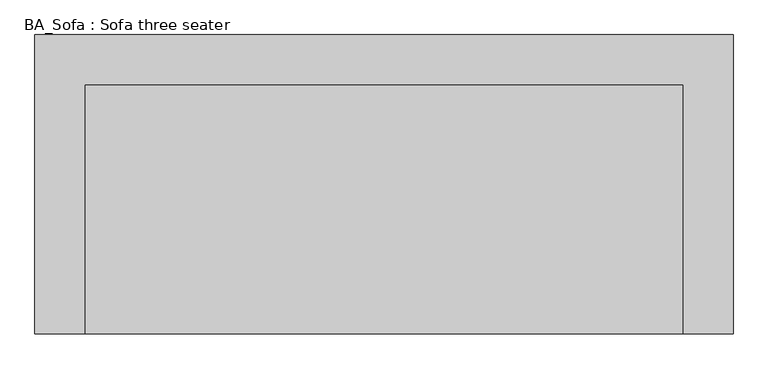
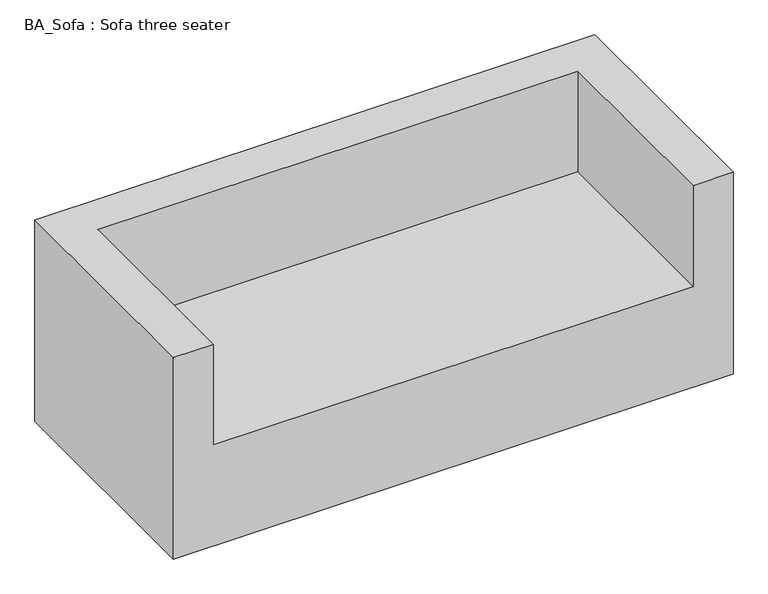
"""IFC4 building model written with IfcOpenShell, lengths in millimetres: furniture geometry, BA_Sofa : Sofa three seater."""

import ifcopenshell
import ifcopenshell.guid

model = None  # the IFC model being written
_history = None  # IfcOwnerHistory: only IFC2X3 demands one
_inside = {}  # id of a spatial element -> (the spatial element, [elements in it])
_under = {}  # id of a project, library or spatial element -> (it, [spatial elements below it])
_declared = {}  # id of a project -> (the project, [libraries it declares])
_typed = {}  # id of a type object -> (the type object, [elements of that type])
_made_of = {}  # id of a material, layer set ... -> (it, [elements and type objects made of it])


def new_model(schema):
    """Start an empty IFC model of exactly this schema.

    Asked for "IFC4X3", IfcOpenShell would pick the latest addendum, in which some entities
    have other attributes; the version numbers below select the first issue.
    IFC2X3 requires an IfcOwnerHistory on every rooted entity: one is made here for all.
    """
    global model, _history
    if schema == "IFC4X3":
        model = ifcopenshell.file(schema_version=(4, 3, 0, 0))
    else:
        model = ifcopenshell.file(schema=schema)
    _inside.clear()
    _under.clear()
    _declared.clear()
    _typed.clear()
    _made_of.clear()
    _history = None
    if model.schema == "IFC2X3":
        org = make("IfcOrganization", Name="unknown")
        user = make(
            "IfcPersonAndOrganization",
            ThePerson=make("IfcPerson", FamilyName="unknown"),
            TheOrganization=org,
        )
        app = make(
            "IfcApplication",
            ApplicationDeveloper=org,
            Version="unknown",
            ApplicationFullName="unknown",
            ApplicationIdentifier="unknown",
        )
        _history = make(
            "IfcOwnerHistory",
            OwningUser=user,
            OwningApplication=app,
            ChangeAction="ADDED",
            CreationDate=0,
        )
    return model


def make(cls, **values):
    """One entity of the class cls with the attributes given. An attribute that is None is left unset."""
    return model.create_entity(
        cls, **{name: value for name, value in values.items() if value is not None}
    )


def rooted(cls, **values):
    """An entity with a GlobalId (a new one), such as an element, a storey or a relation."""
    return make(cls, GlobalId=ifcopenshell.guid.new(), OwnerHistory=_history, **values)


def si_unit(unit_type, name, prefix=None):
    """IfcSIUnit, for example si_unit("LENGTHUNIT", "METRE", prefix="MILLI")."""
    return make("IfcSIUnit", UnitType=unit_type, Prefix=prefix, Name=name)


def assignment(units):
    """IfcUnitAssignment: the units of a project."""
    return None if units is None else make("IfcUnitAssignment", Units=units)


def point(xyz):
    """IfcCartesianPoint."""
    return None if xyz is None else make("IfcCartesianPoint", Coordinates=xyz)


def direction(xyz):
    """IfcDirection."""
    return None if xyz is None else make("IfcDirection", DirectionRatios=xyz)


def frame(location, z_axis=None, x_axis=None):
    """IfcAxis2Placement3D, a coordinate frame: its origin and axes. An axis left out is left unset."""
    return make(
        "IfcAxis2Placement3D",
        Location=point(location),
        Axis=direction(z_axis),
        RefDirection=direction(x_axis),
    )


def origin():
    """The frame at (0, 0, 0) with its axes left unset."""
    return frame((0.0, 0.0, 0.0))


def place(relative_to, where):
    """IfcLocalPlacement: puts the frame where relative to a parent placement (None: the world)."""
    return make(
        "IfcLocalPlacement", PlacementRelTo=relative_to, RelativePlacement=where
    )


def context(
    kind, dimensions, precision=None, world=None, true_north=None, identifier=None
):
    """IfcGeometricRepresentationContext, for example the 3D "Model" context."""
    return make(
        "IfcGeometricRepresentationContext",
        ContextIdentifier=identifier,
        ContextType=kind,
        CoordinateSpaceDimension=dimensions,
        Precision=precision,
        WorldCoordinateSystem=world,
        TrueNorth=true_north,
    )


def project(units=None, contexts=None):
    """IfcProject with its units and contexts."""
    return rooted(
        "IfcProject",
        Name="project",
        RepresentationContexts=contexts,
        UnitsInContext=assignment(units),
    )


def spatial(cls, under=None, at=None, **own):
    """A site, building, storey or space (cls), placed at a placement, below another one or the project."""
    s = rooted(cls, ObjectPlacement=at, **own)
    if under is not None:
        _under.setdefault(under.id(), (under, []))[1].append(s)
    return s


def faces_of(points, faces, orient=None, outer=None):
    """IfcFace entities. A face is a list of loops; a loop is a list of indices into points, from 0.

    orient and outer hold one flag for each loop. By default every Orientation is true, the
    first loop of a face is its IfcFaceOuterBound and the others are IfcFaceBound.
    """
    made = []
    for i, loops in enumerate(faces):
        bounds = []
        for j, loop in enumerate(loops):
            is_outer = j == 0 if outer is None else outer[i][j]
            bounds.append(
                make(
                    "IfcFaceOuterBound" if is_outer else "IfcFaceBound",
                    Bound=make("IfcPolyLoop", Polygon=[points[k] for k in loop]),
                    Orientation=True if orient is None else orient[i][j],
                )
            )
        made.append(make("IfcFace", Bounds=bounds))
    return made


def faceted_brep(points, faces, orient=None, outer=None, voids=None):
    """IfcFacetedBrep: a solid bounded by flat faces; with voids (closed shells), ...WithVoids."""
    shared = [point(p) for p in points]
    hull = make("IfcClosedShell", CfsFaces=faces_of(shared, faces, orient, outer))
    if voids is None:
        return make("IfcFacetedBrep", Outer=hull)
    return make(
        "IfcFacetedBrepWithVoids",
        Outer=hull,
        Voids=[
            make(cls, CfsFaces=faces_of(shared, fs, o, b)) for cls, fs, o, b in voids
        ],
    )


def shape(context_of_items, identifier, shape_type, items):
    """IfcShapeRepresentation: the items that make up one representation, for example the "Body"."""
    return make(
        "IfcShapeRepresentation",
        ContextOfItems=context_of_items,
        RepresentationIdentifier=identifier,
        RepresentationType=shape_type,
        Items=items,
    )


def source(mapping_origin, context_of_items, identifier, shape_type, items):
    """IfcRepresentationMap: a shape defined once, which mapped items show again and again."""
    return make(
        "IfcRepresentationMap",
        MappingOrigin=mapping_origin,
        MappedRepresentation=shape(context_of_items, identifier, shape_type, items),
    )


def transform(
    local_origin,
    x_axis=None,
    y_axis=None,
    z_axis=None,
    scale=None,
    scale2=None,
    scale3=None,
    uniform=True,
):
    """IfcCartesianTransformationOperator3D, or its non-uniform kind. x_axis, y_axis, z_axis: its Axis1, 2, 3."""
    if uniform:
        return make(
            "IfcCartesianTransformationOperator3D",
            Axis1=direction(x_axis),
            Axis2=direction(y_axis),
            LocalOrigin=point(local_origin),
            Scale=scale,
            Axis3=direction(z_axis),
        )
    return make(
        "IfcCartesianTransformationOperator3DnonUniform",
        Axis1=direction(x_axis),
        Axis2=direction(y_axis),
        LocalOrigin=point(local_origin),
        Scale=scale,
        Axis3=direction(z_axis),
        Scale2=scale2,
        Scale3=scale3,
    )


def mapped(mapping_source, mapping_target):
    """IfcMappedItem: shows the shape of a source again, moved by a transform."""
    return make(
        "IfcMappedItem", MappingSource=mapping_source, MappingTarget=mapping_target
    )


def made_of(thing, what):
    """Note that an element or type object is made of a material, layer set ...; save() writes the relation."""
    if what is not None:
        _made_of.setdefault(what.id(), (what, []))[1].append(thing)
    return thing


def element(
    cls,
    number,
    at=None,
    inside=None,
    cuts=None,
    type_object=None,
    material=None,
    context=None,
    identifier="Body",
    shape_type=None,
    held_by="IfcProductDefinitionShape",
    body=None,
    shapes=None,
    **own,
):
    """One element of the class cls, such as IfcWall. Its Tag is "e" and its number.

    at: its placement. inside: the storey or other place that contains it. cuts: it is an
    opening in that element (IfcRelVoidsElement). A single representation is given by context,
    identifier, shape_type and body (its items); several are given by shapes. held_by: the class
    of the entity that holds the representations. save() writes the other relations.
    """
    e = rooted(cls, Tag="e%d" % number, ObjectPlacement=at, **own)
    if body is not None:
        shapes = [shape(context, identifier, shape_type, body)]
    if shapes is not None:
        e.Representation = make(held_by, Representations=shapes)
    if inside is not None:
        _inside.setdefault(inside.id(), (inside, []))[1].append(e)
    if cuts is not None:
        rooted(
            "IfcRelVoidsElement", RelatingBuildingElement=cuts, RelatedOpeningElement=e
        )
    if type_object is not None:
        _typed.setdefault(type_object.id(), (type_object, []))[1].append(e)
    return made_of(e, material)


def aggregate(whole, parts):
    """IfcRelAggregates: a whole, such as a stair, and the parts it consists of."""
    return rooted("IfcRelAggregates", RelatingObject=whole, RelatedObjects=parts)


def save(model, path):
    """Write the relations noted so far, then the file.

    IfcRelAggregates (storeys below a building ...), IfcRelContainedInSpatialStructure (elements
    in a storey), IfcRelDefinesByType, IfcRelAssociatesMaterial and IfcRelDeclares: one each for
    every whole, place, type object, material and project.
    """
    for whole, parts in _under.values():
        aggregate(whole, parts)
    for where, things in _inside.values():
        rooted(
            "IfcRelContainedInSpatialStructure",
            RelatedElements=things,
            RelatingStructure=where,
        )
    for kind, things in _typed.values():
        rooted("IfcRelDefinesByType", RelatedObjects=things, RelatingType=kind)
    for what, things in _made_of.values():
        rooted("IfcRelAssociatesMaterial", RelatedObjects=things, RelatingMaterial=what)
    for by, libraries in _declared.values():
        rooted("IfcRelDeclares", RelatingContext=by, RelatedDefinitions=libraries)
    model.write(path)


def ba_sofa_sofa_three_seater_9d5b51f5(model_context):
    return source(origin(), model_context, "Body", "Brep", [
        faceted_brep([(1050.0, 450.0, 800.0), (-1050.0, 450.0, 800.0), (-1050.0, -450.0, 800.0), (-900.0, -450.0, 800.0), (-900.0, 300.0, 800.0), (900.0, 300.0, 800.0), (900.0, -450.0, 800.0), (1050.0, -450.0, 800.0), (1050.0, 450.0, 0.0), (1050.0, -450.0, 0.0), (-1050.0, -450.0, 0.0), (-1050.0, 450.0, 0.0), (900.0, -450.0, 400.0), (-900.0, -450.0, 400.0), (-900.0, 300.0, 400.0), (900.0, 300.0, 400.0)], [[[0, 1, 2, 3, 4, 5, 6, 7]], [[8, 9, 10, 11]], [[1, 0, 8, 11]], [[2, 1, 11, 10]], [[3, 2, 10, 9, 7, 6, 12, 13]], [[4, 3, 13, 14]], [[5, 4, 14, 15]], [[6, 5, 15, 12]], [[0, 7, 9, 8]], [[13, 12, 15, 14]]]),
    ])


if __name__ == "__main__":
    model = new_model("IFC4")
    model_context = context("Model", 3, world=origin())
    ifc_project = project(units=[si_unit("LENGTHUNIT", "METRE", prefix="MILLI")], contexts=[model_context])
    site = spatial("IfcSite", under=ifc_project)
    building = spatial("IfcBuilding", under=site)
    placement = place(None, origin())
    ba_sofa_sofa_three_seater_shape = ba_sofa_sofa_three_seater_9d5b51f5(model_context)
    element("IfcFurniture", 1, ObjectType="BA_Sofa : Sofa three seater", at=placement, inside=building, context=model_context, shape_type="MappedRepresentation", body=[
        mapped(ba_sofa_sofa_three_seater_shape, transform((0.0, 0.0, 0.0), x_axis=(1.0, 0.0, 0.0), y_axis=(0.0, 1.0, 0.0), z_axis=(0.0, 0.0, 1.0))),
    ])
    save(model, "model.ifc")

# Revit data of these elements
# Type "BA_Sofa : Sofa three seater"
#   height = 800 mm
#   width = 900 mm
#   length = 2100 mm
#   Default Elevation = 0
# Element 1 (IfcFurniture, "BA_Sofa : Sofa three seater")
#   Materials on its faces: "Default"
# Materials
#   "Default": class "Generic", colour RGB 255 255 255, transparency 0, Cost = 0
